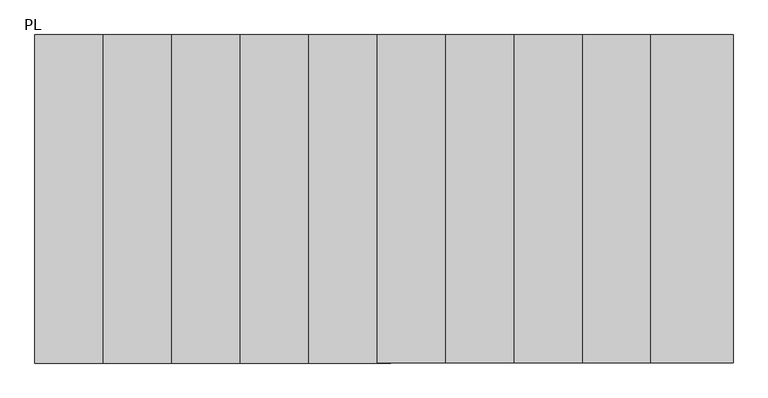
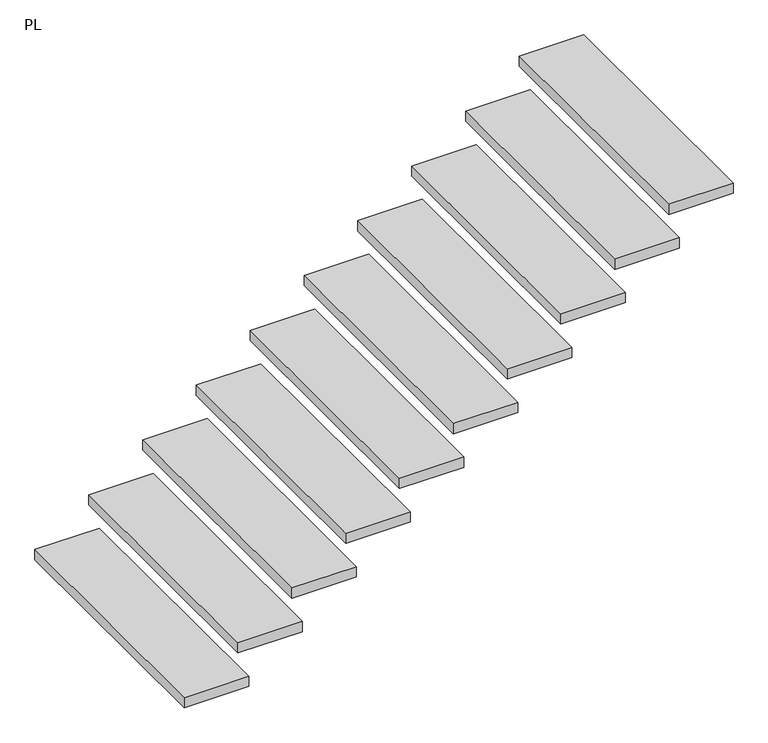
"""IFC4 building model written with IfcOpenShell, lengths in millimetres: stair flight geometry, PL."""

import ifcopenshell
import ifcopenshell.guid

model = None  # the IFC model being written
_history = None  # IfcOwnerHistory: only IFC2X3 demands one
_inside = {}  # id of a spatial element -> (the spatial element, [elements in it])
_under = {}  # id of a project, library or spatial element -> (it, [spatial elements below it])
_declared = {}  # id of a project -> (the project, [libraries it declares])
_typed = {}  # id of a type object -> (the type object, [elements of that type])
_made_of = {}  # id of a material, layer set ... -> (it, [elements and type objects made of it])


def new_model(schema):
    """Start an empty IFC model of exactly this schema.

    Asked for "IFC4X3", IfcOpenShell would pick the latest addendum, in which some entities
    have other attributes; the version numbers below select the first issue.
    IFC2X3 requires an IfcOwnerHistory on every rooted entity: one is made here for all.
    """
    global model, _history
    if schema == "IFC4X3":
        model = ifcopenshell.file(schema_version=(4, 3, 0, 0))
    else:
        model = ifcopenshell.file(schema=schema)
    _inside.clear()
    _under.clear()
    _declared.clear()
    _typed.clear()
    _made_of.clear()
    _history = None
    if model.schema == "IFC2X3":
        org = make("IfcOrganization", Name="unknown")
        user = make(
            "IfcPersonAndOrganization",
            ThePerson=make("IfcPerson", FamilyName="unknown"),
            TheOrganization=org,
        )
        app = make(
            "IfcApplication",
            ApplicationDeveloper=org,
            Version="unknown",
            ApplicationFullName="unknown",
            ApplicationIdentifier="unknown",
        )
        _history = make(
            "IfcOwnerHistory",
            OwningUser=user,
            OwningApplication=app,
            ChangeAction="ADDED",
            CreationDate=0,
        )
    return model


def make(cls, **values):
    """One entity of the class cls with the attributes given. An attribute that is None is left unset."""
    return model.create_entity(
        cls, **{name: value for name, value in values.items() if value is not None}
    )


def rooted(cls, **values):
    """An entity with a GlobalId (a new one), such as an element, a storey or a relation."""
    return make(cls, GlobalId=ifcopenshell.guid.new(), OwnerHistory=_history, **values)


def si_unit(unit_type, name, prefix=None):
    """IfcSIUnit, for example si_unit("LENGTHUNIT", "METRE", prefix="MILLI")."""
    return make("IfcSIUnit", UnitType=unit_type, Prefix=prefix, Name=name)


def assignment(units):
    """IfcUnitAssignment: the units of a project."""
    return None if units is None else make("IfcUnitAssignment", Units=units)


def point(xyz):
    """IfcCartesianPoint."""
    return None if xyz is None else make("IfcCartesianPoint", Coordinates=xyz)


def direction(xyz):
    """IfcDirection."""
    return None if xyz is None else make("IfcDirection", DirectionRatios=xyz)


def frame(location, z_axis=None, x_axis=None):
    """IfcAxis2Placement3D, a coordinate frame: its origin and axes. An axis left out is left unset."""
    return make(
        "IfcAxis2Placement3D",
        Location=point(location),
        Axis=direction(z_axis),
        RefDirection=direction(x_axis),
    )


def origin():
    """The frame at (0, 0, 0) with its axes left unset."""
    return frame((0.0, 0.0, 0.0))


def place(relative_to, where):
    """IfcLocalPlacement: puts the frame where relative to a parent placement (None: the world)."""
    return make(
        "IfcLocalPlacement", PlacementRelTo=relative_to, RelativePlacement=where
    )


def context(
    kind, dimensions, precision=None, world=None, true_north=None, identifier=None
):
    """IfcGeometricRepresentationContext, for example the 3D "Model" context."""
    return make(
        "IfcGeometricRepresentationContext",
        ContextIdentifier=identifier,
        ContextType=kind,
        CoordinateSpaceDimension=dimensions,
        Precision=precision,
        WorldCoordinateSystem=world,
        TrueNorth=true_north,
    )


def project(units=None, contexts=None):
    """IfcProject with its units and contexts."""
    return rooted(
        "IfcProject",
        Name="project",
        RepresentationContexts=contexts,
        UnitsInContext=assignment(units),
    )


def spatial(cls, under=None, at=None, **own):
    """A site, building, storey or space (cls), placed at a placement, below another one or the project."""
    s = rooted(cls, ObjectPlacement=at, **own)
    if under is not None:
        _under.setdefault(under.id(), (under, []))[1].append(s)
    return s


def polyline(points):
    """IfcPolyline through the points."""
    return make("IfcPolyline", Points=[point(p) for p in points])


def outline(outer, holes=None, kind="AREA"):
    """IfcArbitraryClosedProfileDef: a profile drawn as a closed curve; with holes, ...WithVoids."""
    if holes is None:
        return make("IfcArbitraryClosedProfileDef", ProfileType=kind, OuterCurve=outer)
    return make(
        "IfcArbitraryProfileDefWithVoids",
        ProfileType=kind,
        OuterCurve=outer,
        InnerCurves=holes,
    )


def extrude(swept, where, along, depth):
    """IfcExtrudedAreaSolid: the profile swept, set in the frame where, extruded along a direction by depth."""
    return make(
        "IfcExtrudedAreaSolid",
        SweptArea=swept,
        Position=where,
        ExtrudedDirection=direction(along),
        Depth=depth,
    )


def shape(context_of_items, identifier, shape_type, items):
    """IfcShapeRepresentation: the items that make up one representation, for example the "Body"."""
    return make(
        "IfcShapeRepresentation",
        ContextOfItems=context_of_items,
        RepresentationIdentifier=identifier,
        RepresentationType=shape_type,
        Items=items,
    )


def source(mapping_origin, context_of_items, identifier, shape_type, items):
    """IfcRepresentationMap: a shape defined once, which mapped items show again and again."""
    return make(
        "IfcRepresentationMap",
        MappingOrigin=mapping_origin,
        MappedRepresentation=shape(context_of_items, identifier, shape_type, items),
    )


def transform(
    local_origin,
    x_axis=None,
    y_axis=None,
    z_axis=None,
    scale=None,
    scale2=None,
    scale3=None,
    uniform=True,
):
    """IfcCartesianTransformationOperator3D, or its non-uniform kind. x_axis, y_axis, z_axis: its Axis1, 2, 3."""
    if uniform:
        return make(
            "IfcCartesianTransformationOperator3D",
            Axis1=direction(x_axis),
            Axis2=direction(y_axis),
            LocalOrigin=point(local_origin),
            Scale=scale,
            Axis3=direction(z_axis),
        )
    return make(
        "IfcCartesianTransformationOperator3DnonUniform",
        Axis1=direction(x_axis),
        Axis2=direction(y_axis),
        LocalOrigin=point(local_origin),
        Scale=scale,
        Axis3=direction(z_axis),
        Scale2=scale2,
        Scale3=scale3,
    )


def mapped(mapping_source, mapping_target):
    """IfcMappedItem: shows the shape of a source again, moved by a transform."""
    return make(
        "IfcMappedItem", MappingSource=mapping_source, MappingTarget=mapping_target
    )


def made_of(thing, what):
    """Note that an element or type object is made of a material, layer set ...; save() writes the relation."""
    if what is not None:
        _made_of.setdefault(what.id(), (what, []))[1].append(thing)
    return thing


def element(
    cls,
    number,
    at=None,
    inside=None,
    cuts=None,
    type_object=None,
    material=None,
    context=None,
    identifier="Body",
    shape_type=None,
    held_by="IfcProductDefinitionShape",
    body=None,
    shapes=None,
    **own,
):
    """One element of the class cls, such as IfcWall. Its Tag is "e" and its number.

    at: its placement. inside: the storey or other place that contains it. cuts: it is an
    opening in that element (IfcRelVoidsElement). A single representation is given by context,
    identifier, shape_type and body (its items); several are given by shapes. held_by: the class
    of the entity that holds the representations. save() writes the other relations.
    """
    e = rooted(cls, Tag="e%d" % number, ObjectPlacement=at, **own)
    if body is not None:
        shapes = [shape(context, identifier, shape_type, body)]
    if shapes is not None:
        e.Representation = make(held_by, Representations=shapes)
    if inside is not None:
        _inside.setdefault(inside.id(), (inside, []))[1].append(e)
    if cuts is not None:
        rooted(
            "IfcRelVoidsElement", RelatingBuildingElement=cuts, RelatedOpeningElement=e
        )
    if type_object is not None:
        _typed.setdefault(type_object.id(), (type_object, []))[1].append(e)
    return made_of(e, material)


def aggregate(whole, parts):
    """IfcRelAggregates: a whole, such as a stair, and the parts it consists of."""
    return rooted("IfcRelAggregates", RelatingObject=whole, RelatedObjects=parts)


def save(model, path):
    """Write the relations noted so far, then the file.

    IfcRelAggregates (storeys below a building ...), IfcRelContainedInSpatialStructure (elements
    in a storey), IfcRelDefinesByType, IfcRelAssociatesMaterial and IfcRelDeclares: one each for
    every whole, place, type object, material and project.
    """
    for whole, parts in _under.values():
        aggregate(whole, parts)
    for where, things in _inside.values():
        rooted(
            "IfcRelContainedInSpatialStructure",
            RelatedElements=things,
            RelatingStructure=where,
        )
    for kind, things in _typed.values():
        rooted("IfcRelDefinesByType", RelatedObjects=things, RelatingType=kind)
    for what, things in _made_of.values():
        rooted("IfcRelAssociatesMaterial", RelatedObjects=things, RelatingMaterial=what)
    for by, libraries in _declared.values():
        rooted("IfcRelDeclares", RelatingContext=by, RelatedDefinitions=libraries)
    model.write(path)


def pl_d6e87e92(model_context):
    return source(origin(), model_context, "Body", "SweptSolid", [
        extrude(outline(polyline([(4109.5374538, 36032.6086665), (3809.5374538, 36032.6086665), (3809.5374538, 37232.6086665), (4109.5374538, 37232.6086665), (4109.5374538, 36032.6086665)])), frame((0.0, 0.0, 2731.7901873), z_axis=(0.0, 0.0, 1.0), x_axis=(1.0, 0.0, 0.0)), (0.0, 0.0, 1.0), 50.0),
        extrude(outline(polyline([(4359.5374538, 36032.6086665), (4059.5374538, 36032.6086665), (4059.5374538, 37232.6086665), (4359.5374538, 37232.6086665), (4359.5374538, 36032.6086665)])), frame((0.0, 0.0, 2913.6083692), z_axis=(0.0, 0.0, 1.0), x_axis=(1.0, 0.0, 0.0)), (0.0, 0.0, 1.0), 50.0),
        extrude(outline(polyline([(4609.5374538, 36032.6086665), (4309.5374538, 36032.6086665), (4309.5374538, 37232.6086665), (4609.5374538, 37232.6086665), (4609.5374538, 36032.6086665)])), frame((0.0, 0.0, 3095.426551), z_axis=(0.0, 0.0, 1.0), x_axis=(1.0, 0.0, 0.0)), (0.0, 0.0, 1.0), 50.0),
        extrude(outline(polyline([(4859.5374538, 36032.6086665), (4559.5374538, 36032.6086665), (4559.5374538, 37232.6086665), (4859.5374538, 37232.6086665), (4859.5374538, 36032.6086665)])), frame((0.0, 0.0, 3277.2447328), z_axis=(0.0, 0.0, 1.0), x_axis=(1.0, 0.0, 0.0)), (0.0, 0.0, 1.0), 50.0),
        extrude(outline(polyline([(5109.5374538, 36032.6086665), (4809.5374538, 36032.6086665), (4809.5374538, 37232.6086665), (5109.5374538, 37232.6086665), (5109.5374538, 36032.6086665)])), frame((0.0, 0.0, 3459.0629146), z_axis=(0.0, 0.0, 1.0), x_axis=(1.0, 0.0, 0.0)), (0.0, 0.0, 1.0), 50.0),
        extrude(outline(polyline([(5359.5374538, 36032.6086665), (5059.5374538, 36032.6086665), (5059.5374538, 37232.6086665), (5359.5374538, 37232.6086665), (5359.5374538, 36032.6086665)])), frame((0.0, 0.0, 3640.8810964), z_axis=(0.0, 0.0, 1.0), x_axis=(1.0, 0.0, 0.0)), (0.0, 0.0, 1.0), 50.0),
        extrude(outline(polyline([(5609.5374538, 36032.6086665), (5309.5374538, 36032.6086665), (5309.5374538, 37232.6086665), (5609.5374538, 37232.6086665), (5609.5374538, 36032.6086665)])), frame((0.0, 0.0, 3822.6992783), z_axis=(0.0, 0.0, 1.0), x_axis=(1.0, 0.0, 0.0)), (0.0, 0.0, 1.0), 50.0),
        extrude(outline(polyline([(5859.5374538, 36032.6086665), (5559.5374538, 36032.6086665), (5559.5374538, 37232.6086665), (5859.5374538, 37232.6086665), (5859.5374538, 36032.6086665)])), frame((0.0, 0.0, 4004.5174601), z_axis=(0.0, 0.0, 1.0), x_axis=(1.0, 0.0, 0.0)), (0.0, 0.0, 1.0), 50.0),
        extrude(outline(polyline([(6109.5374538, 36032.6086665), (5809.5374538, 36032.6086665), (5809.5374538, 37232.6086665), (6109.5374538, 37232.6086665), (6109.5374538, 36032.6086665)])), frame((0.0, 0.0, 4186.3356419), z_axis=(0.0, 0.0, 1.0), x_axis=(1.0, 0.0, 0.0)), (0.0, 0.0, 1.0), 50.0),
        extrude(outline(polyline([(6359.5374538, 36032.6086665), (6059.5374538, 36032.6086665), (6059.5374538, 37232.6086665), (6359.5374538, 37232.6086665), (6359.5374538, 36032.6086665)])), frame((0.0, 0.0, 4368.1538237), z_axis=(0.0, 0.0, 1.0), x_axis=(1.0, 0.0, 0.0)), (0.0, 0.0, 1.0), 50.0),
    ])


if __name__ == "__main__":
    model = new_model("IFC4")
    model_context = context("Model", 3, world=origin())
    ifc_project = project(units=[si_unit("LENGTHUNIT", "METRE", prefix="MILLI")], contexts=[model_context])
    site = spatial("IfcSite", under=ifc_project)
    building = spatial("IfcBuilding", under=site)
    placement = place(None, origin())
    pl_shape = pl_d6e87e92(model_context)
    element("IfcStairFlight", 1, ObjectType="PL", at=placement, inside=building, context=model_context, shape_type="MappedRepresentation", body=[
        mapped(pl_shape, transform((0.0, 0.0, 0.0), x_axis=(1.0, 0.0, 0.0), y_axis=(0.0, 1.0, 0.0), z_axis=(0.0, 0.0, 1.0))),
    ])
    save(model, "model.ifc")
